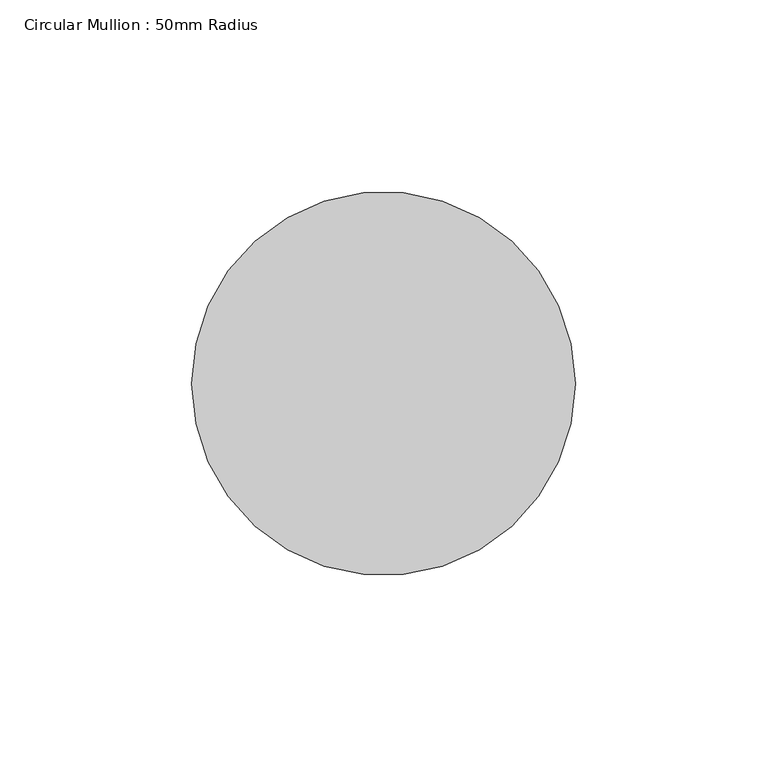
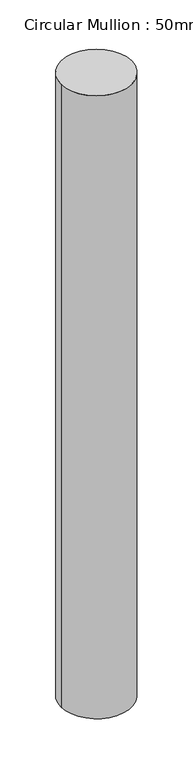
"""IFC4 building model written with IfcOpenShell, lengths in millimetres: member geometry, Circular Mullion : 50mm Radius."""

from ifc_helpers import new_model, si_unit, point, frame, origin, origin_2d, place, context, project, spatial, circle_curve, trimmed, segment, composite_curve, outline, extrude, source, transform, mapped, element, save


def circular_mullion_50mm_radius_c7fce439(model_context):
    return source(origin(), model_context, "Body", "SweptSolid", [
        extrude(outline(composite_curve([segment(trimmed(circle_curve(origin_2d(), 50.0), [point((50.0, 0.0))], [point((-50.0, 0.0))], False, "CARTESIAN"), True, "CONTINUOUS"), segment(trimmed(circle_curve(origin_2d(), 50.0), [point((-50.0, 0.0))], [point((50.0, 0.0))], False, "CARTESIAN"), True, "CONTINUOUS")], self_intersect=False)), frame((0.0, 0.0, -933.777889), z_axis=(0.0, 0.0, 1.0), x_axis=(1.0, 0.0, 0.0)), (0.0, 0.0, 1.0), 933.777889),
    ])


if __name__ == "__main__":
    model = new_model("IFC4")
    model_context = context("Model", 3, world=origin())
    ifc_project = project(units=[si_unit("LENGTHUNIT", "METRE", prefix="MILLI")], contexts=[model_context])
    site = spatial("IfcSite", under=ifc_project)
    building = spatial("IfcBuilding", under=site)
    placement = place(None, origin())
    circular_mullion_50mm_radius_shape = circular_mullion_50mm_radius_c7fce439(model_context)
    element("IfcMember", 1, ObjectType="Circular Mullion : 50mm Radius", at=placement, inside=building, context=model_context, shape_type="MappedRepresentation", body=[
        mapped(circular_mullion_50mm_radius_shape, transform((0.0, 0.0, 0.0), x_axis=(1.0, 0.0, 0.0), y_axis=(0.0, 1.0, 0.0), z_axis=(0.0, 0.0, 1.0))),
    ])
    save(model, "model.ifc")

# Revit data of these elements
# Type "Circular Mullion : 50mm Radius"
#   built-in parameter 1007350 = 0.164042 (stored number, unit not read)
# Element 1 (IfcMember, "Circular Mullion : 50mm Radius")
#   Materials on its faces: "Aluminium"
# Materials
#   "Aluminium": class "Metal", colour RGB 247 247 247, transparency 0, Description = "Aluminium 6061", Cost = 0
